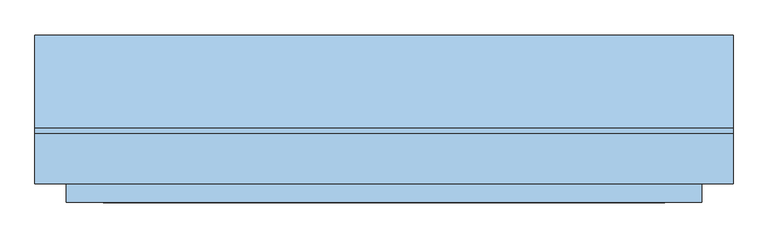
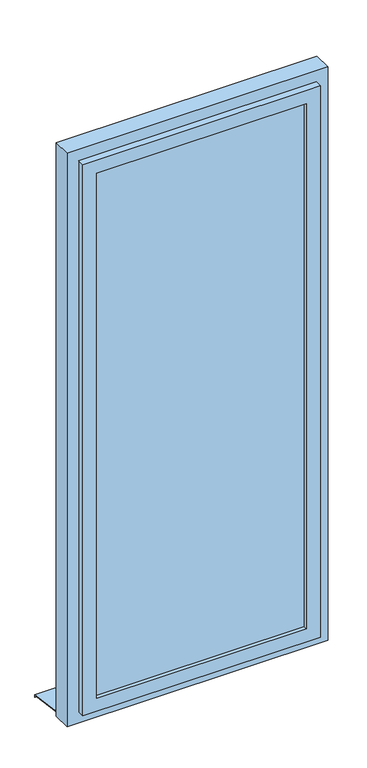
"""IFC4 building model written with IfcOpenShell, lengths in millimetres: window geometry, Fenstertür 1-flg : 1.80 x  3,1."""

from ifc_helpers import new_model, si_unit, frame, origin, place, context, project, spatial, polyline, outline, extrude, faceted_brep, source, transform, mapped, element, save


def window_971a6d9a(model_context):
    return source(origin(), model_context, "Body", "SolidModel", [
        extrude(outline(polyline([(2600.0, 560.0), (2600.0, -560.0), (0.0, -560.0), (0.0, 560.0), (2600.0, 560.0)]), holes=[polyline([(2520.0, 480.0), (80.0, 480.0), (80.0, -480.0), (2520.0, -480.0), (2520.0, 480.0)])]), frame((0.0, 91.3106168, 0.0), z_axis=(0.0, 1.0, 0.0), x_axis=(0.0, 0.0, 1.0)), (0.0, 0.0, 1.0), 80.0),
        faceted_brep([(510.0, 91.3106168, 2550.0), (510.0, 61.3106168, 2550.0), (510.0, 61.3106168, 50.0), (510.0, 91.3106168, 50.0), (-510.0, 61.3106168, 2550.0), (-510.0, 61.3106168, 50.0), (450.0, 61.3106168, 110.0), (-450.0, 61.3106168, 110.0), (-450.0, 61.3106168, 2490.0), (450.0, 61.3106168, 2490.0), (-510.0, 91.3106168, 50.0), (-510.0, 91.3106168, 2550.0), (480.0, 91.3106168, 2520.0), (-480.0, 91.3106168, 2520.0), (-480.0, 91.3106168, 80.0), (480.0, 91.3106168, 80.0), (480.0, 121.3106168, 2520.0), (480.0, 121.3106168, 80.0), (-480.0, 121.3106168, 80.0), (-480.0, 121.3106168, 2520.0), (450.0, 121.3106168, 2490.0), (-450.0, 121.3106168, 2490.0), (-450.0, 121.3106168, 110.0), (450.0, 121.3106168, 110.0)], [[[0, 1, 2, 3]], [[1, 4, 5, 2], [6, 7, 8, 9]], [[3, 2, 5, 10]], [[3, 10, 11, 0], [12, 13, 14, 15]], [[16, 12, 15, 17]], [[17, 15, 14, 18]], [[17, 18, 19, 16], [20, 21, 22, 23]], [[9, 20, 23, 6]], [[6, 23, 22, 7]], [[10, 5, 4, 11]], [[18, 14, 13, 19]], [[7, 22, 21, 8]], [[11, 4, 1, 0]], [[19, 13, 12, 16]], [[8, 21, 20, 9]]]),
        extrude(outline(polyline([(181.3327711, 20.0), (330.0, 0.0), (330.0, -10.0), (328.0, -10.0), (328.0, -1.6395366), (181.1346891, 18.0), (171.3106168, 18.0), (171.3106168, 20.0), (181.3327711, 20.0)])), frame((-560.0, 0.0, 0.0), z_axis=(1.0, 0.0, 0.0), x_axis=(0.0, 1.0, 0.0)), (0.0, 0.0, 1.0), 1120.0),
        extrude(outline(polyline([(450.0, 76.3106168), (-450.0, 76.3106168), (-450.0, 106.3106168), (450.0, 106.3106168), (450.0, 76.3106168)])), frame((0.0, 0.0, 110.0), z_axis=(0.0, 0.0, 1.0), x_axis=(1.0, 0.0, 0.0)), (0.0, 0.0, 1.0), 2380.0),
    ])


if __name__ == "__main__":
    model = new_model("IFC4")
    model_context = context("Model", 3, world=origin())
    ifc_project = project(units=[si_unit("LENGTHUNIT", "METRE", prefix="MILLI")], contexts=[model_context])
    site = spatial("IfcSite", under=ifc_project)
    building = spatial("IfcBuilding", under=site)
    placement = place(None, origin())
    window_shape = window_971a6d9a(model_context)
    element("IfcWindow", 1, ObjectType="Fenstertür 1-flg : 1.80 x  3,1", at=placement, inside=building, context=model_context, shape_type="MappedRepresentation", body=[
        mapped(window_shape, transform((0.0, 0.0, 0.0), x_axis=(1.0, 0.0, 0.0), y_axis=(0.0, 1.0, 0.0), z_axis=(0.0, 0.0, 1.0))),
    ])
    save(model, "model.ifc")

# Revit data of these elements
# Type "Fenstertür 1-flg : 1.80 x  3,1"
#   Type Mark = "51"
#   Operation = "SinglePanel"
#   Construction Type Id = "GSP4R"
#   Keynote = "16.05.01"
#   Analytic Construction = "1/8 Zoll Pilkington-Verglasung einfach"
#   Visual Light Transmittance = 0.9
#   Thermal Resistance (R) = 0.1491 (m²·K)/W
#   Solar Heat Gain Coefficient = 0.86
#   Rough Width = 1.120 m
#   Rough Height = 2.600 m
#   Heat Transfer Coefficient (U) = 6.7069 W/(m²·K)
#   Rahmentiefe = 0.080 m
#   Rahmenhöhe - unten = 0.080 m
#   Rahmenhöhe - oben = 0.080 m
#   Rahmenbreite = 0.080 m
#   Height = 2.600 m
#   Tiefe Flügel = 0.060 m
#   Flügelbreite = 0.060 m
#   Einbautiefe (von außen) [instance default] = 0.080 m
#   Width = 1.120 m
#   Kippflügel [instance default] = yes
#   Drehflügel im Grundriss darstellen [instance default] = yes
#   Drehflügel 1 [instance default] = yes
#   Rahmen 1 [instance default] = none
#   Glas [instance default] = none
#   Flügel [instance default] = none
#   Fensterbank Außenseite [instance default] = none
#   Wall Closure = (empty or 0)
# Element 1 (IfcWindow, "Fenstertür 1-flg : 1.80 x  3,1")
#   Einbautiefe (von außen) = 0.128689 m
#   Materials on its faces: "Kunststoff - Weiß", "Glas"
# Materials
#   "Kunststoff - Weiß": class "Kunststoff", colour RGB 249 249 249, transparency 0, Cost = 0
#   "Glas": class "Glas", colour RGB 0 0 255, transparency 0.75, Comments = "Render-Darstellung nicht aktualisiert ", Cost = 0
